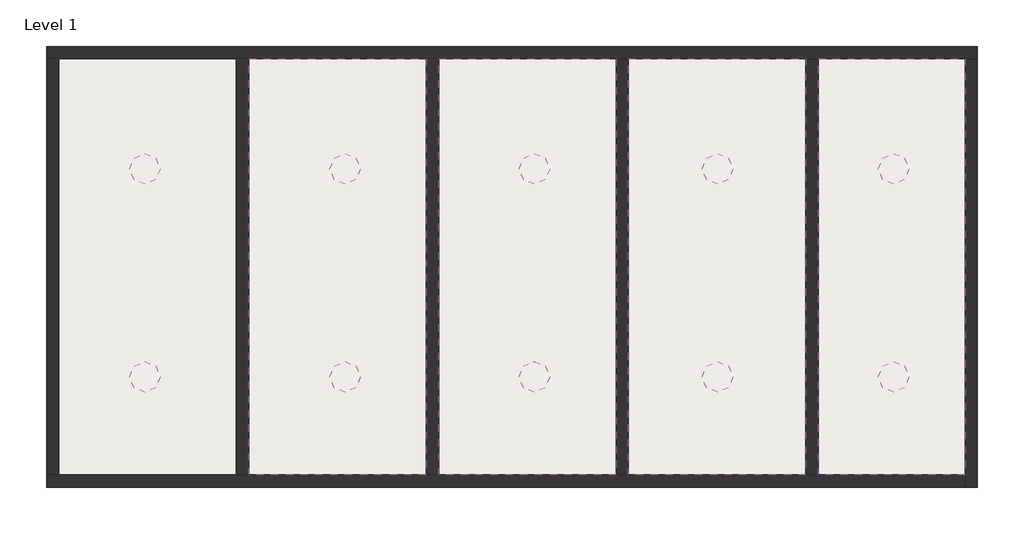
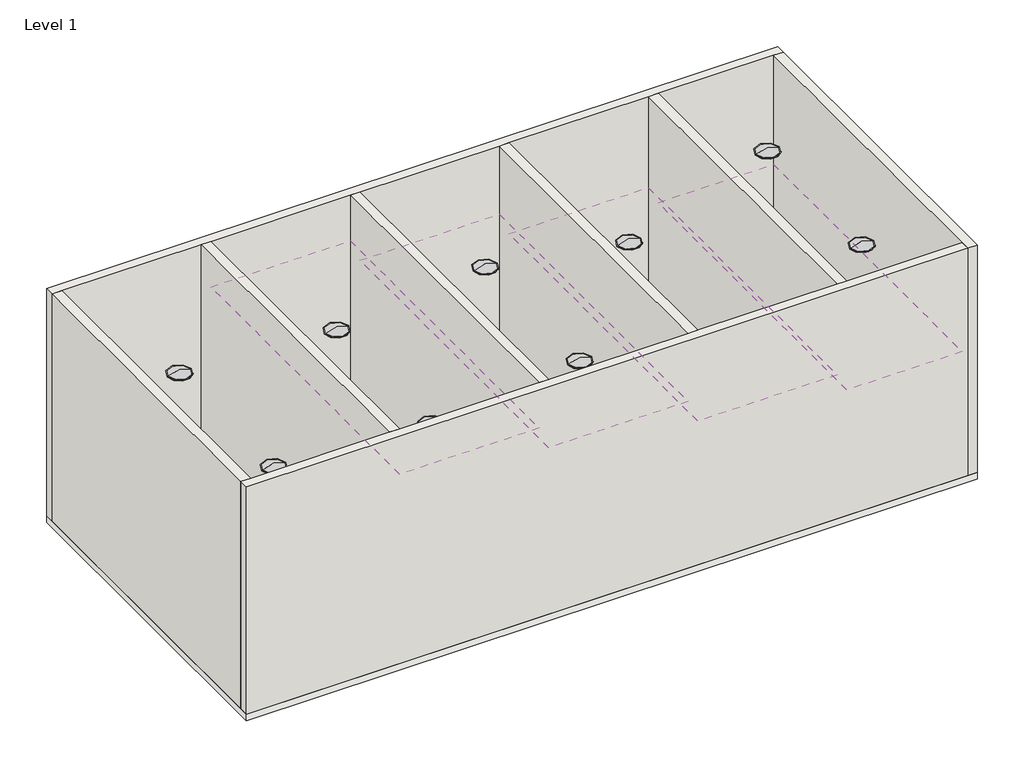
# One storey: 10 light fixtures, 8 walls, 4 coverings, 1 slab.
"""IFC4 building model written with IfcOpenShell, lengths in millimetres."""

import ifcopenshell
import ifcopenshell.guid

model = None  # the IFC model being written
_history = None  # IfcOwnerHistory: only IFC2X3 demands one
_inside = {}  # id of a spatial element -> (the spatial element, [elements in it])
_under = {}  # id of a project, library or spatial element -> (it, [spatial elements below it])
_declared = {}  # id of a project -> (the project, [libraries it declares])
_typed = {}  # id of a type object -> (the type object, [elements of that type])
_made_of = {}  # id of a material, layer set ... -> (it, [elements and type objects made of it])


def new_model(schema):
    """Start an empty IFC model of exactly this schema.

    Asked for "IFC4X3", IfcOpenShell would pick the latest addendum, in which some entities
    have other attributes; the version numbers below select the first issue.
    IFC2X3 requires an IfcOwnerHistory on every rooted entity: one is made here for all.
    """
    global model, _history
    if schema == "IFC4X3":
        model = ifcopenshell.file(schema_version=(4, 3, 0, 0))
    else:
        model = ifcopenshell.file(schema=schema)
    _inside.clear()
    _under.clear()
    _declared.clear()
    _typed.clear()
    _made_of.clear()
    _history = None
    if model.schema == "IFC2X3":
        org = make("IfcOrganization", Name="unknown")
        user = make(
            "IfcPersonAndOrganization",
            ThePerson=make("IfcPerson", FamilyName="unknown"),
            TheOrganization=org,
        )
        app = make(
            "IfcApplication",
            ApplicationDeveloper=org,
            Version="unknown",
            ApplicationFullName="unknown",
            ApplicationIdentifier="unknown",
        )
        _history = make(
            "IfcOwnerHistory",
            OwningUser=user,
            OwningApplication=app,
            ChangeAction="ADDED",
            CreationDate=0,
        )
    return model


def make(cls, **values):
    """One entity of the class cls with the attributes given. An attribute that is None is left unset."""
    return model.create_entity(
        cls, **{name: value for name, value in values.items() if value is not None}
    )


def rooted(cls, **values):
    """An entity with a GlobalId (a new one), such as an element, a storey or a relation."""
    return make(cls, GlobalId=ifcopenshell.guid.new(), OwnerHistory=_history, **values)


def si_unit(unit_type, name, prefix=None):
    """IfcSIUnit, for example si_unit("LENGTHUNIT", "METRE", prefix="MILLI")."""
    return make("IfcSIUnit", UnitType=unit_type, Prefix=prefix, Name=name)


def assignment(units):
    """IfcUnitAssignment: the units of a project."""
    return None if units is None else make("IfcUnitAssignment", Units=units)


def point(xyz):
    """IfcCartesianPoint."""
    return None if xyz is None else make("IfcCartesianPoint", Coordinates=xyz)


def direction(xyz):
    """IfcDirection."""
    return None if xyz is None else make("IfcDirection", DirectionRatios=xyz)


def frame(location, z_axis=None, x_axis=None):
    """IfcAxis2Placement3D, a coordinate frame: its origin and axes. An axis left out is left unset."""
    return make(
        "IfcAxis2Placement3D",
        Location=point(location),
        Axis=direction(z_axis),
        RefDirection=direction(x_axis),
    )


def frame_2d(location, x_axis=None):
    """IfcAxis2Placement2D, a coordinate frame in the plane: its origin and x axis."""
    return make(
        "IfcAxis2Placement2D", Location=point(location), RefDirection=direction(x_axis)
    )


def origin():
    """The frame at (0, 0, 0) with its axes left unset."""
    return frame((0.0, 0.0, 0.0))


def origin_with_axes():
    """The frame at (0, 0, 0) with the z axis (0, 0, 1) and the x axis (1, 0, 0) written out."""
    return frame((0.0, 0.0, 0.0), z_axis=(0.0, 0.0, 1.0), x_axis=(1.0, 0.0, 0.0))


def origin_2d():
    """The frame at (0, 0) in the plane with its x axis left unset."""
    return frame_2d((0.0, 0.0))


def place(relative_to, where):
    """IfcLocalPlacement: puts the frame where relative to a parent placement (None: the world)."""
    return make(
        "IfcLocalPlacement", PlacementRelTo=relative_to, RelativePlacement=where
    )


def context(
    kind, dimensions, precision=None, world=None, true_north=None, identifier=None
):
    """IfcGeometricRepresentationContext, for example the 3D "Model" context."""
    return make(
        "IfcGeometricRepresentationContext",
        ContextIdentifier=identifier,
        ContextType=kind,
        CoordinateSpaceDimension=dimensions,
        Precision=precision,
        WorldCoordinateSystem=world,
        TrueNorth=true_north,
    )


def project(units=None, contexts=None):
    """IfcProject with its units and contexts."""
    return rooted(
        "IfcProject",
        Name="project",
        RepresentationContexts=contexts,
        UnitsInContext=assignment(units),
    )


def spatial(cls, under=None, at=None, **own):
    """A site, building, storey or space (cls), placed at a placement, below another one or the project."""
    s = rooted(cls, ObjectPlacement=at, **own)
    if under is not None:
        _under.setdefault(under.id(), (under, []))[1].append(s)
    return s


def polyline(points):
    """IfcPolyline through the points."""
    return make("IfcPolyline", Points=[point(p) for p in points])


def circle_curve(where, radius):
    """IfcCircle in the frame where."""
    return make("IfcCircle", Position=where, Radius=radius)


def ellipse_curve(where, semi_axis1, semi_axis2):
    """IfcEllipse in the frame where."""
    return make(
        "IfcEllipse", Position=where, SemiAxis1=semi_axis1, SemiAxis2=semi_axis2
    )


def trimmed(basis, trim1, trim2, sense, master):
    """IfcTrimmedCurve: the piece of a basis curve between two trims."""
    return make(
        "IfcTrimmedCurve",
        BasisCurve=basis,
        Trim1=trim1,
        Trim2=trim2,
        SenseAgreement=sense,
        MasterRepresentation=master,
    )


def segment(curve, same_sense, transition):
    """IfcCompositeCurveSegment."""
    return make(
        "IfcCompositeCurveSegment",
        Transition=transition,
        SameSense=same_sense,
        ParentCurve=curve,
    )


def composite_curve(segments, self_intersect=None):
    """IfcCompositeCurve: segments joined end to end."""
    return make("IfcCompositeCurve", Segments=segments, SelfIntersect=self_intersect)


def outline(outer, holes=None, kind="AREA"):
    """IfcArbitraryClosedProfileDef: a profile drawn as a closed curve; with holes, ...WithVoids."""
    if holes is None:
        return make("IfcArbitraryClosedProfileDef", ProfileType=kind, OuterCurve=outer)
    return make(
        "IfcArbitraryProfileDefWithVoids",
        ProfileType=kind,
        OuterCurve=outer,
        InnerCurves=holes,
    )


def extrude(swept, where, along, depth):
    """IfcExtrudedAreaSolid: the profile swept, set in the frame where, extruded along a direction by depth."""
    return make(
        "IfcExtrudedAreaSolid",
        SweptArea=swept,
        Position=where,
        ExtrudedDirection=direction(along),
        Depth=depth,
    )


def faces_of(points, faces, orient=None, outer=None):
    """IfcFace entities. A face is a list of loops; a loop is a list of indices into points, from 0.

    orient and outer hold one flag for each loop. By default every Orientation is true, the
    first loop of a face is its IfcFaceOuterBound and the others are IfcFaceBound.
    """
    made = []
    for i, loops in enumerate(faces):
        bounds = []
        for j, loop in enumerate(loops):
            is_outer = j == 0 if outer is None else outer[i][j]
            bounds.append(
                make(
                    "IfcFaceOuterBound" if is_outer else "IfcFaceBound",
                    Bound=make("IfcPolyLoop", Polygon=[points[k] for k in loop]),
                    Orientation=True if orient is None else orient[i][j],
                )
            )
        made.append(make("IfcFace", Bounds=bounds))
    return made


def faceted_brep(points, faces, orient=None, outer=None, voids=None):
    """IfcFacetedBrep: a solid bounded by flat faces; with voids (closed shells), ...WithVoids."""
    shared = [point(p) for p in points]
    hull = make("IfcClosedShell", CfsFaces=faces_of(shared, faces, orient, outer))
    if voids is None:
        return make("IfcFacetedBrep", Outer=hull)
    return make(
        "IfcFacetedBrepWithVoids",
        Outer=hull,
        Voids=[
            make(cls, CfsFaces=faces_of(shared, fs, o, b)) for cls, fs, o, b in voids
        ],
    )


def shape(context_of_items, identifier, shape_type, items):
    """IfcShapeRepresentation: the items that make up one representation, for example the "Body"."""
    return make(
        "IfcShapeRepresentation",
        ContextOfItems=context_of_items,
        RepresentationIdentifier=identifier,
        RepresentationType=shape_type,
        Items=items,
    )


def source(mapping_origin, context_of_items, identifier, shape_type, items):
    """IfcRepresentationMap: a shape defined once, which mapped items show again and again."""
    return make(
        "IfcRepresentationMap",
        MappingOrigin=mapping_origin,
        MappedRepresentation=shape(context_of_items, identifier, shape_type, items),
    )


def transform(
    local_origin,
    x_axis=None,
    y_axis=None,
    z_axis=None,
    scale=None,
    scale2=None,
    scale3=None,
    uniform=True,
):
    """IfcCartesianTransformationOperator3D, or its non-uniform kind. x_axis, y_axis, z_axis: its Axis1, 2, 3."""
    if uniform:
        return make(
            "IfcCartesianTransformationOperator3D",
            Axis1=direction(x_axis),
            Axis2=direction(y_axis),
            LocalOrigin=point(local_origin),
            Scale=scale,
            Axis3=direction(z_axis),
        )
    return make(
        "IfcCartesianTransformationOperator3DnonUniform",
        Axis1=direction(x_axis),
        Axis2=direction(y_axis),
        LocalOrigin=point(local_origin),
        Scale=scale,
        Axis3=direction(z_axis),
        Scale2=scale2,
        Scale3=scale3,
    )


def mapped(mapping_source, mapping_target):
    """IfcMappedItem: shows the shape of a source again, moved by a transform."""
    return make(
        "IfcMappedItem", MappingSource=mapping_source, MappingTarget=mapping_target
    )


def made_of(thing, what):
    """Note that an element or type object is made of a material, layer set ...; save() writes the relation."""
    if what is not None:
        _made_of.setdefault(what.id(), (what, []))[1].append(thing)
    return thing


def element(
    cls,
    number,
    at=None,
    inside=None,
    cuts=None,
    type_object=None,
    material=None,
    context=None,
    identifier="Body",
    shape_type=None,
    held_by="IfcProductDefinitionShape",
    body=None,
    shapes=None,
    **own,
):
    """One element of the class cls, such as IfcWall. Its Tag is "e" and its number.

    at: its placement. inside: the storey or other place that contains it. cuts: it is an
    opening in that element (IfcRelVoidsElement). A single representation is given by context,
    identifier, shape_type and body (its items); several are given by shapes. held_by: the class
    of the entity that holds the representations. save() writes the other relations.
    """
    e = rooted(cls, Tag="e%d" % number, ObjectPlacement=at, **own)
    if body is not None:
        shapes = [shape(context, identifier, shape_type, body)]
    if shapes is not None:
        e.Representation = make(held_by, Representations=shapes)
    if inside is not None:
        _inside.setdefault(inside.id(), (inside, []))[1].append(e)
    if cuts is not None:
        rooted(
            "IfcRelVoidsElement", RelatingBuildingElement=cuts, RelatedOpeningElement=e
        )
    if type_object is not None:
        _typed.setdefault(type_object.id(), (type_object, []))[1].append(e)
    return made_of(e, material)


def aggregate(whole, parts):
    """IfcRelAggregates: a whole, such as a stair, and the parts it consists of."""
    return rooted("IfcRelAggregates", RelatingObject=whole, RelatedObjects=parts)


def save(model, path):
    """Write the relations noted so far, then the file.

    IfcRelAggregates (storeys below a building ...), IfcRelContainedInSpatialStructure (elements
    in a storey), IfcRelDefinesByType, IfcRelAssociatesMaterial and IfcRelDeclares: one each for
    every whole, place, type object, material and project.
    """
    for whole, parts in _under.values():
        aggregate(whole, parts)
    for where, things in _inside.values():
        rooted(
            "IfcRelContainedInSpatialStructure",
            RelatedElements=things,
            RelatingStructure=where,
        )
    for kind, things in _typed.values():
        rooted("IfcRelDefinesByType", RelatedObjects=things, RelatingType=kind)
    for what, things in _made_of.values():
        rooted("IfcRelAssociatesMaterial", RelatedObjects=things, RelatingMaterial=what)
    for by, libraries in _declared.values():
        rooted("IfcRelDeclares", RelatingContext=by, RelatedDefinitions=libraries)
    model.write(path)


def plane_surface(at):
    """IfcPlane: the flat surface through the origin of the frame at, square to its z axis."""
    return make("IfcPlane", Position=at)


def revolved_surface(curve, axis_point, axis_direction):
    """IfcSurfaceOfRevolution: the curve turned about the line through axis_point along axis_direction."""
    return make(
        "IfcSurfaceOfRevolution",
        SweptCurve=make("IfcArbitraryOpenProfileDef", ProfileType="CURVE", Curve=curve),
        AxisPosition=make("IfcAxis1Placement", Location=point(axis_point), Axis=direction(axis_direction)),
    )


def advanced_brep(points, edges, surfaces, faces):
    """IfcAdvancedBrep: a solid bounded by faces that lie on surfaces and meet in shared edges.

    An edge is (start, end): straight between two places in points (the first is 0);
    or (start, end, curve); or (start, end, curve, False) where it runs against its curve.
    A face is (place in surfaces, loops), or (place, loops, False) where it looks against
    its surface's normal. A loop lists edges by number (the first is 1), with a minus sign
    where the edge is run from its end to its start. The first loop is the outer one.
    """
    corners = [point(p) for p in points]
    vertices = [make("IfcVertexPoint", VertexGeometry=c) for c in corners]
    made = []
    for start, end, *more in edges:
        made.append(
            make(
                "IfcEdgeCurve",
                EdgeStart=vertices[start],
                EdgeEnd=vertices[end],
                EdgeGeometry=more[0] if more else make("IfcPolyline", Points=[corners[start], corners[end]]),
                SameSense=more[1] if len(more) > 1 else True,
            )
        )
    hull = []
    for where, loops, *sense in faces:
        bounds = []
        for j, loop in enumerate(loops):
            ring = [make("IfcOrientedEdge", EdgeElement=made[abs(k) - 1], Orientation=k > 0) for k in loop]
            bounds.append(
                make(
                    "IfcFaceOuterBound" if j == 0 else "IfcFaceBound",
                    Bound=make("IfcEdgeLoop", EdgeList=ring),
                    Orientation=True,
                )
            )
        hull.append(make("IfcAdvancedFace", Bounds=bounds, FaceSurface=surfaces[where], SameSense=sense[0] if sense else True))
    return make("IfcAdvancedBrep", Outer=make("IfcClosedShell", CfsFaces=hull))


def downlight_downlight_e6a68a7d(model_context):
    return source(origin(), model_context, "Body", "SolidModel", [
        advanced_brep(
        [(-230.0, 0.0, 0.0), (230.0, 0.0, 0.0), (0.0, 0.0, 0.0), (0.0, 0.0, 70.3180567)],
        [
            (0, 1, circle_curve(frame((0.0, 0.0, 0.0), z_axis=(0.0, 0.0, -1.0), x_axis=(1.0, 0.0, 0.0)), 230.0)),
            (1, 2),
            (2, 0),
            (1, 0, circle_curve(frame((0.0, 0.0, 0.0), z_axis=(0.0, 0.0, -1.0), x_axis=(1.0, 0.0, 0.0)), 230.0)),
            (3, 1, circle_curve(frame((13.1969865, 0.0, -297.8236248), z_axis=(0.0, 1.0, 0.0), x_axis=(1.0, 0.0, 0.0)), 368.3781456)),
            (0, 3, circle_curve(frame((-13.1969865, 0.0, -297.8236248), z_axis=(0.0, 1.0, 0.0), x_axis=(-1.0, 0.0, 0.0)), 368.3781456)),
        ],
        [
            plane_surface(frame((0.0, 0.0, 0.0), z_axis=(0.0, 0.0, -1.0), x_axis=(1.0, 0.0, 0.0))),
            revolved_surface(trimmed(ellipse_curve(frame((13.1969865, 0.0, -297.8236248), z_axis=(0.0, -1.0, 0.0), x_axis=(1.0, 0.0, 0.0)), 368.3781456, 368.3781456), [point((230.0, 0.0, 0.0))], [point((0.0, 0.0, 70.3180567))], True, "CARTESIAN"), (0.0, 0.0, 2194.0651339), (0.0, 0.0, 1.0)),
        ],
        [
            (0, [[1, 2, 3]]),
            (0, [[4, -3, -2]]),
            (1, [[5, -1, 6]]),
            (1, [[-6, -4, -5]]),
        ],
    ),
        extrude(outline(composite_curve([segment(trimmed(circle_curve(origin_2d(), 250.0), [point((-250.0, 0.0))], [point((250.0, 0.0))], False, "CARTESIAN"), True, "CONTINUOUS"), segment(trimmed(circle_curve(origin_2d(), 250.0), [point((250.0, 0.0))], [point((-250.0, 0.0))], False, "CARTESIAN"), True, "CONTINUOUS")], self_intersect=False)), frame((0.0, 0.0, -10.1537533), z_axis=(0.0, 0.0, 1.0), x_axis=(1.0, 0.0, 0.0)), (0.0, 0.0, 1.0), 10.1537533),
    ])


model = new_model("IFC4")

# Units and contexts
model_context = context("Model", 3, world=origin())
ifc_project = project(units=[si_unit("LENGTHUNIT", "METRE", prefix="MILLI")], contexts=[model_context])

# Site, building, storey
site = spatial("IfcSite", under=ifc_project)
building = spatial("IfcBuilding", under=site)
storey = spatial("IfcBuildingStorey", under=building, Name="Level 1", Elevation=0.0)

# Coverings
placement = place(None, origin())
element("IfcCovering", 1, ObjectType="Plain", at=placement, inside=storey, context=model_context, shape_type="SweptSolid", body=[
    extrude(outline(polyline([(4711.6370984, -2494.7382368), (4711.6370984, 4305.2617632), (7111.6370984, 4305.2617632), (7111.6370984, -2494.7382368), (4711.6370984, -2494.7382368)])), frame((0.0, 0.0, 2600.0), z_axis=(0.0, 0.0, 1.0), x_axis=(1.0, 0.0, 0.0)), (0.0, 0.0, 1.0), 57.0),
])
element("IfcCovering", 2, ObjectType="Plain", at=placement, inside=storey, context=model_context, shape_type="SweptSolid", body=[
    extrude(outline(polyline([(1611.6370984, -2494.7382368), (1611.6370984, 4305.2617632), (4511.6370984, 4305.2617632), (4511.6370984, -2494.7382368), (1611.6370984, -2494.7382368)])), frame((0.0, 0.0, 3000.0), z_axis=(0.0, 0.0, 1.0), x_axis=(1.0, 0.0, 0.0)), (0.0, 0.0, 1.0), 57.0),
])
element("IfcCovering", 3, ObjectType="Plain", at=placement, inside=storey, context=model_context, shape_type="SweptSolid", body=[
    extrude(outline(polyline([(-1488.3629016, -2494.7382368), (-1488.3629016, 4305.2617632), (1411.6370984, 4305.2617632), (1411.6370984, -2494.7382368), (-1488.3629016, -2494.7382368)])), frame((0.0, 0.0, 3500.0), z_axis=(0.0, 0.0, 1.0), x_axis=(1.0, 0.0, 0.0)), (0.0, 0.0, 1.0), 57.0),
])
element("IfcCovering", 4, ObjectType="Plain", at=placement, inside=storey, context=model_context, shape_type="SweptSolid", body=[
    extrude(outline(polyline([(-4588.3629016, -2494.7382368), (-4588.3629016, 4305.2617632), (-1688.3629016, 4305.2617632), (-1688.3629016, -2494.7382368), (-4588.3629016, -2494.7382368)])), frame((0.0, 0.0, 4000.0), z_axis=(0.0, 0.0, 1.0), x_axis=(1.0, 0.0, 0.0)), (0.0, 0.0, 1.0), 57.0),
])

# Light fixtures
downlight_downlight_shape = downlight_downlight_e6a68a7d(model_context)
element("IfcLightFixture", 5, ObjectType="Downlight : Downlight", at=placement, inside=storey, context=model_context, shape_type="MappedRepresentation", body=[
    mapped(downlight_downlight_shape, transform((-6282.0675101, -895.1572455, 3800.0), x_axis=(1.0, 0.0, 0.0), y_axis=(0.0, 1.0, 0.0), z_axis=(0.0, 0.0, 1.0))),
])
element("IfcLightFixture", 6, ObjectType="Downlight : Downlight", at=placement, inside=storey, context=model_context, shape_type="MappedRepresentation", body=[
    mapped(downlight_downlight_shape, transform((-6282.0675101, 2504.8427545, 3800.0), x_axis=(1.0, 0.0, 0.0), y_axis=(0.0, 1.0, 0.0), z_axis=(0.0, 0.0, 1.0))),
])
element("IfcLightFixture", 7, ObjectType="Downlight : Downlight", at=placement, inside=storey, context=model_context, shape_type="MappedRepresentation", body=[
    mapped(downlight_downlight_shape, transform((-3013.7777439, -895.1572455, 3600.0), x_axis=(1.0, 0.0, 0.0), y_axis=(0.0, 1.0, 0.0), z_axis=(0.0, 0.0, 1.0))),
])
element("IfcLightFixture", 8, ObjectType="Downlight : Downlight", at=placement, inside=storey, context=model_context, shape_type="MappedRepresentation", body=[
    mapped(downlight_downlight_shape, transform((-3013.7777439, 2504.8427545, 3600.0), x_axis=(1.0, 0.0, 0.0), y_axis=(0.0, 1.0, 0.0), z_axis=(0.0, 0.0, 1.0))),
])
element("IfcLightFixture", 9, ObjectType="Downlight : Downlight", at=placement, inside=storey, context=model_context, shape_type="MappedRepresentation", body=[
    mapped(downlight_downlight_shape, transform((76.5388311, -895.1572455, 3900.0), x_axis=(1.0, 0.0, 0.0), y_axis=(0.0, 1.0, 0.0), z_axis=(0.0, 0.0, 1.0))),
])
element("IfcLightFixture", 10, ObjectType="Downlight : Downlight", at=placement, inside=storey, context=model_context, shape_type="MappedRepresentation", body=[
    mapped(downlight_downlight_shape, transform((76.5388311, 2504.8427545, 3900.0), x_axis=(1.0, 0.0, 0.0), y_axis=(0.0, 1.0, 0.0), z_axis=(0.0, 0.0, 1.0))),
])
element("IfcLightFixture", 11, ObjectType="Downlight : Downlight", at=placement, inside=storey, context=model_context, shape_type="MappedRepresentation", body=[
    mapped(downlight_downlight_shape, transform((3067.3545284, -895.1572455, 3400.0), x_axis=(1.0, 0.0, 0.0), y_axis=(0.0, 1.0, 0.0), z_axis=(0.0, 0.0, 1.0))),
])
element("IfcLightFixture", 12, ObjectType="Downlight : Downlight", at=placement, inside=storey, context=model_context, shape_type="MappedRepresentation", body=[
    mapped(downlight_downlight_shape, transform((3067.3545284, 2504.8427545, 3400.0), x_axis=(1.0, 0.0, 0.0), y_axis=(0.0, 1.0, 0.0), z_axis=(0.0, 0.0, 1.0))),
])
element("IfcLightFixture", 13, ObjectType="Downlight : Downlight", at=placement, inside=storey, context=model_context, shape_type="MappedRepresentation", body=[
    mapped(downlight_downlight_shape, transform((5942.4423645, -895.1572455, 4400.0), x_axis=(1.0, 0.0, 0.0), y_axis=(0.0, 1.0, 0.0), z_axis=(0.0, 0.0, 1.0))),
])
element("IfcLightFixture", 14, ObjectType="Downlight : Downlight", at=placement, inside=storey, context=model_context, shape_type="MappedRepresentation", body=[
    mapped(downlight_downlight_shape, transform((5942.4423645, 2504.8427545, 4400.0), x_axis=(1.0, 0.0, 0.0), y_axis=(0.0, 1.0, 0.0), z_axis=(0.0, 0.0, 1.0))),
])

# Slab
element("IfcSlab", 15, ObjectType="Generic 150mm", at=placement, inside=storey, context=model_context, shape_type="SweptSolid", body=[
    extrude(outline(polyline([(7311.6370984, 4505.2617632), (7311.6370984, -2694.7382368), (-7888.3629016, -2694.7382368), (-7888.3629016, 4505.2617632), (7311.6370984, 4505.2617632)])), frame((0.0, 0.0, -150.0), z_axis=(0.0, 0.0, 1.0), x_axis=(1.0, 0.0, 0.0)), (0.0, 0.0, 1.0), 150.0),
])

# Walls
element("IfcWall", 16, ObjectType="Generic - 200mm", at=placement, inside=storey, context=model_context, shape_type="Brep", body=[
    faceted_brep([(-7888.3629016, 4305.2617632, 0.0), (-7688.3629016, 4305.2617632, 0.0), (-4788.3629016, 4305.2617632, 0.0), (-4588.3629016, 4305.2617632, 0.0), (-1688.3629016, 4305.2617632, 0.0), (-1488.3629016, 4305.2617632, 0.0), (1411.6370984, 4305.2617632, 0.0), (1611.6370984, 4305.2617632, 0.0), (4511.6370984, 4305.2617632, 0.0), (4711.6370984, 4305.2617632, 0.0), (7111.6370984, 4305.2617632, 0.0), (7311.6370984, 4305.2617632, 0.0), (7311.6370984, 4305.2617632, 5000.0), (7111.6370984, 4305.2617632, 5000.0), (4711.6370984, 4305.2617632, 5000.0), (4511.6370984, 4305.2617632, 5000.0), (1611.6370984, 4305.2617632, 5000.0), (1411.6370984, 4305.2617632, 5000.0), (-1488.3629016, 4305.2617632, 5000.0), (-1688.3629016, 4305.2617632, 5000.0), (-4588.3629016, 4305.2617632, 5000.0), (-4788.3629016, 4305.2617632, 5000.0), (-7688.3629016, 4305.2617632, 5000.0), (-7888.3629016, 4305.2617632, 5000.0), (-7888.3629016, 4505.2617632, 0.0), (-7888.3629016, 4505.2617632, 5000.0), (7311.6370984, 4505.2617632, 5000.0), (7311.6370984, 4505.2617632, 0.0)], [[[0, 1, 2, 3, 4, 5, 6, 7, 8, 9, 10, 11, 12, 13, 14, 15, 16, 17, 18, 19, 20, 21, 22, 23]], [[24, 25, 26, 27]], [[11, 10, 9, 8, 7, 6, 5, 4, 3, 2, 1, 0, 24, 27]], [[23, 22, 21, 20, 19, 18, 17, 16, 15, 14, 13, 12, 26, 25]], [[12, 11, 27, 26]], [[0, 23, 25, 24]]]),
])
element("IfcWall", 17, ObjectType="Generic - 200mm", at=placement, inside=storey, context=model_context, shape_type="Brep", body=[
    faceted_brep([(7111.6370984, 4305.2617632, 0.0), (7111.6370984, -2494.7382368, 0.0), (7111.6370984, -2694.7382368, 0.0), (7111.6370984, -2694.7382368, 5000.0), (7111.6370984, -2494.7382368, 5000.0), (7111.6370984, 4305.2617632, 5000.0), (7311.6370984, 4305.2617632, 0.0), (7311.6370984, 4305.2617632, 5000.0), (7311.6370984, -2694.7382368, 5000.0), (7311.6370984, -2694.7382368, 0.0)], [[[0, 1, 2, 3, 4, 5]], [[6, 7, 8, 9]], [[2, 1, 0, 6, 9]], [[5, 4, 3, 8, 7]], [[0, 5, 7, 6]], [[3, 2, 9, 8]]]),
])
element("IfcWall", 18, ObjectType="Generic - 200mm", at=placement, inside=storey, context=model_context, shape_type="Brep", body=[
    faceted_brep([(7111.6370984, -2494.7382368, 0.0), (4711.6370984, -2494.7382368, 0.0), (4511.6370984, -2494.7382368, 0.0), (1611.6370984, -2494.7382368, 0.0), (1411.6370984, -2494.7382368, 0.0), (-1488.3629016, -2494.7382368, 0.0), (-1688.3629016, -2494.7382368, 0.0), (-4588.3629016, -2494.7382368, 0.0), (-4788.3629016, -2494.7382368, 0.0), (-7688.3629016, -2494.7382368, 0.0), (-7888.3629016, -2494.7382368, 0.0), (-7888.3629016, -2494.7382368, 5000.0), (-7688.3629016, -2494.7382368, 5000.0), (-4788.3629016, -2494.7382368, 5000.0), (-4588.3629016, -2494.7382368, 5000.0), (-1688.3629016, -2494.7382368, 5000.0), (-1488.3629016, -2494.7382368, 5000.0), (1411.6370984, -2494.7382368, 5000.0), (1611.6370984, -2494.7382368, 5000.0), (4511.6370984, -2494.7382368, 5000.0), (4711.6370984, -2494.7382368, 5000.0), (7111.6370984, -2494.7382368, 5000.0), (7111.6370984, -2694.7382368, 0.0), (7111.6370984, -2694.7382368, 5000.0), (-7888.3629016, -2694.7382368, 5000.0), (-7888.3629016, -2694.7382368, 0.0)], [[[0, 1, 2, 3, 4, 5, 6, 7, 8, 9, 10, 11, 12, 13, 14, 15, 16, 17, 18, 19, 20, 21]], [[22, 23, 24, 25]], [[10, 9, 8, 7, 6, 5, 4, 3, 2, 1, 0, 22, 25]], [[21, 20, 19, 18, 17, 16, 15, 14, 13, 12, 11, 24, 23]], [[0, 21, 23, 22]], [[11, 10, 25, 24]]]),
])
element("IfcWall", 19, ObjectType="Generic - 200mm", at=placement, inside=storey, context=model_context, shape_type="SweptSolid", body=[
    extrude(outline(polyline([(-7688.3629016, 4305.2617632), (-7688.3629016, -2494.7382368), (-7888.3629016, -2494.7382368), (-7888.3629016, 4305.2617632), (-7688.3629016, 4305.2617632)])), origin_with_axes(), (0.0, 0.0, 1.0), 5000.0),
])
element("IfcWall", 20, ObjectType="Generic - 200mm", at=placement, inside=storey, context=model_context, shape_type="SweptSolid", body=[
    extrude(outline(polyline([(-4788.3629016, -2494.7382368), (-4788.3629016, 4305.2617632), (-4588.3629016, 4305.2617632), (-4588.3629016, -2494.7382368), (-4788.3629016, -2494.7382368)])), origin_with_axes(), (0.0, 0.0, 1.0), 5000.0),
])
element("IfcWall", 21, ObjectType="Generic - 200mm", at=placement, inside=storey, context=model_context, shape_type="SweptSolid", body=[
    extrude(outline(polyline([(-1688.3629016, -2494.7382368), (-1688.3629016, 4305.2617632), (-1488.3629016, 4305.2617632), (-1488.3629016, -2494.7382368), (-1688.3629016, -2494.7382368)])), origin_with_axes(), (0.0, 0.0, 1.0), 5000.0),
])
element("IfcWall", 22, ObjectType="Generic - 200mm", at=placement, inside=storey, context=model_context, shape_type="SweptSolid", body=[
    extrude(outline(polyline([(1411.6370984, -2494.7382368), (1411.6370984, 4305.2617632), (1611.6370984, 4305.2617632), (1611.6370984, -2494.7382368), (1411.6370984, -2494.7382368)])), origin_with_axes(), (0.0, 0.0, 1.0), 5000.0),
])
element("IfcWall", 23, ObjectType="Generic - 200mm", at=placement, inside=storey, context=model_context, shape_type="SweptSolid", body=[
    extrude(outline(polyline([(4511.6370984, -2494.7382368), (4511.6370984, 4305.2617632), (4711.6370984, 4305.2617632), (4711.6370984, -2494.7382368), (4511.6370984, -2494.7382368)])), origin_with_axes(), (0.0, 0.0, 1.0), 5000.0),
])

save(model, "model.ifc")

# Revit data of these elements
# Project information
#   Project Issue Date = "Issue Date"
#   Project Status = "Project Status"
#   Client Name = "Owner"
#   Project Address = "Enter address here"
#   Project Name = "Project Name"
#   Project Number = "0001"
# Type "Plain"
#   built-in parameter 1002203 = 1 (stored number, unit not read)
#   built-in parameter 1002202 = 1 (stored number, unit not read)
#   Layers, outside or top first: 0.045 m "Metal Stud Layer" (function 1); 0.012 m "Gypsum Wall Board" (function 1)
# Type "Downlight : Downlight"
#   Default Elevation = 0
# Type "Generic 150mm"
#   Function = 0
#   Layers, outside or top first: 0.15 m no material (function 1)
# Type "Generic - 200mm"
#   Layers, outside or top first: 0.2 m no material (function 1)
# Element 1 (IfcCovering, "Plain")
#   Height Offset From Level = 2.6 m
#   Phase Created = New Construction
#   Materials on its faces: "Gypsum Wall Board", "Metal Stud Layer"
# Element 2 (IfcCovering, "Plain")
#   Height Offset From Level = 3 m
#   Phase Created = New Construction
#   Materials on its faces: "Gypsum Wall Board", "Metal Stud Layer"
# Element 3 (IfcCovering, "Plain")
#   Height Offset From Level = 3.5 m
#   Phase Created = New Construction
#   Materials on its faces: "Gypsum Wall Board", "Metal Stud Layer"
# Element 4 (IfcCovering, "Plain")
#   Height Offset From Level = 4 m
#   Phase Created = New Construction
#   Materials on its faces: "Gypsum Wall Board", "Metal Stud Layer"
# Element 5 (IfcLightFixture, "Downlight : Downlight")
#   Mark = "23"
#   Phase Created = New Construction
# Element 6 (IfcLightFixture, "Downlight : Downlight")
#   Mark = "24"
#   Phase Created = New Construction
# Element 7 (IfcLightFixture, "Downlight : Downlight")
#   Mark = "25"
#   Phase Created = New Construction
# Element 8 (IfcLightFixture, "Downlight : Downlight")
#   Mark = "26"
#   Phase Created = New Construction
# Element 9 (IfcLightFixture, "Downlight : Downlight")
#   Mark = "27"
#   Phase Created = New Construction
# Element 10 (IfcLightFixture, "Downlight : Downlight")
#   Mark = "28"
#   Phase Created = New Construction
# Element 11 (IfcLightFixture, "Downlight : Downlight")
#   Mark = "29"
#   Phase Created = New Construction
# Element 12 (IfcLightFixture, "Downlight : Downlight")
#   Mark = "30"
#   Phase Created = New Construction
# Element 13 (IfcLightFixture, "Downlight : Downlight")
#   Mark = "31"
#   Phase Created = New Construction
# Element 14 (IfcLightFixture, "Downlight : Downlight")
#   Mark = "32"
#   Phase Created = New Construction
# Element 15 (IfcSlab, "Generic 150mm")
#   Height Offset From Level = 0 m
#   Phase Created = New Construction
#   Materials on its faces: "Default Floor"
# Elements 16, 17, 18, 19, 20, 21, 22, 23 (IfcWall, "Generic - 200mm")
#   Top Offset = 0 m
#   Base Offset = 0 m
#   wall height = 5 m
#   Phase Created = New Construction
#   Base Constraint = Level 1
#   Top Constraint = Level 2
#   Materials on its faces: "Default Wall"
# Materials
#   "Metal Stud Layer": class "Metal", colour RGB 127 127 127, transparency 0, Description = "Light gauge steel framing, thermal air layer", Cost = 0
#   "Gypsum Wall Board": class "Generic", colour RGB 249 249 249, transparency 0, Description = "Gypsum Wall Board", Cost = 0
#   "Default Floor": class "Miscellaneous", colour RGB 127 127 127, transparency 0, Cost = 0
#   "Default Wall": class "Miscellaneous", colour RGB 128 128 128, transparency 0, Cost = 0
